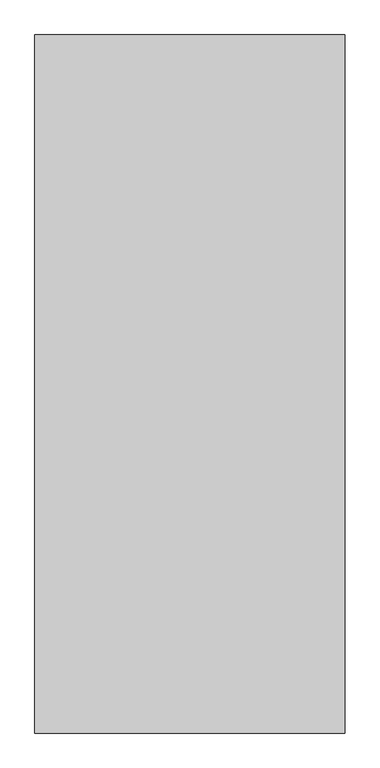
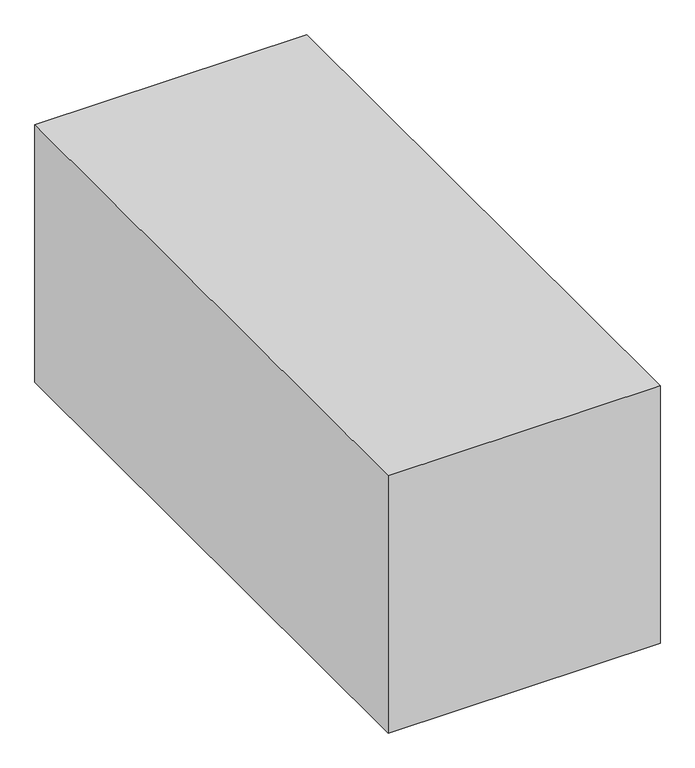
"""IFC4 building model written with IfcOpenShell, lengths in millimetres: proxy geometry, Space Planning Box_hec : Space Planning Box_hec."""

import ifcopenshell
import ifcopenshell.guid

model = None  # the IFC model being written
_history = None  # IfcOwnerHistory: only IFC2X3 demands one
_inside = {}  # id of a spatial element -> (the spatial element, [elements in it])
_under = {}  # id of a project, library or spatial element -> (it, [spatial elements below it])
_declared = {}  # id of a project -> (the project, [libraries it declares])
_typed = {}  # id of a type object -> (the type object, [elements of that type])
_made_of = {}  # id of a material, layer set ... -> (it, [elements and type objects made of it])


def new_model(schema):
    """Start an empty IFC model of exactly this schema.

    Asked for "IFC4X3", IfcOpenShell would pick the latest addendum, in which some entities
    have other attributes; the version numbers below select the first issue.
    IFC2X3 requires an IfcOwnerHistory on every rooted entity: one is made here for all.
    """
    global model, _history
    if schema == "IFC4X3":
        model = ifcopenshell.file(schema_version=(4, 3, 0, 0))
    else:
        model = ifcopenshell.file(schema=schema)
    _inside.clear()
    _under.clear()
    _declared.clear()
    _typed.clear()
    _made_of.clear()
    _history = None
    if model.schema == "IFC2X3":
        org = make("IfcOrganization", Name="unknown")
        user = make(
            "IfcPersonAndOrganization",
            ThePerson=make("IfcPerson", FamilyName="unknown"),
            TheOrganization=org,
        )
        app = make(
            "IfcApplication",
            ApplicationDeveloper=org,
            Version="unknown",
            ApplicationFullName="unknown",
            ApplicationIdentifier="unknown",
        )
        _history = make(
            "IfcOwnerHistory",
            OwningUser=user,
            OwningApplication=app,
            ChangeAction="ADDED",
            CreationDate=0,
        )
    return model


def make(cls, **values):
    """One entity of the class cls with the attributes given. An attribute that is None is left unset."""
    return model.create_entity(
        cls, **{name: value for name, value in values.items() if value is not None}
    )


def rooted(cls, **values):
    """An entity with a GlobalId (a new one), such as an element, a storey or a relation."""
    return make(cls, GlobalId=ifcopenshell.guid.new(), OwnerHistory=_history, **values)


def si_unit(unit_type, name, prefix=None):
    """IfcSIUnit, for example si_unit("LENGTHUNIT", "METRE", prefix="MILLI")."""
    return make("IfcSIUnit", UnitType=unit_type, Prefix=prefix, Name=name)


def assignment(units):
    """IfcUnitAssignment: the units of a project."""
    return None if units is None else make("IfcUnitAssignment", Units=units)


def point(xyz):
    """IfcCartesianPoint."""
    return None if xyz is None else make("IfcCartesianPoint", Coordinates=xyz)


def direction(xyz):
    """IfcDirection."""
    return None if xyz is None else make("IfcDirection", DirectionRatios=xyz)


def frame(location, z_axis=None, x_axis=None):
    """IfcAxis2Placement3D, a coordinate frame: its origin and axes. An axis left out is left unset."""
    return make(
        "IfcAxis2Placement3D",
        Location=point(location),
        Axis=direction(z_axis),
        RefDirection=direction(x_axis),
    )


def origin():
    """The frame at (0, 0, 0) with its axes left unset."""
    return frame((0.0, 0.0, 0.0))


def origin_with_axes():
    """The frame at (0, 0, 0) with the z axis (0, 0, 1) and the x axis (1, 0, 0) written out."""
    return frame((0.0, 0.0, 0.0), z_axis=(0.0, 0.0, 1.0), x_axis=(1.0, 0.0, 0.0))


def place(relative_to, where):
    """IfcLocalPlacement: puts the frame where relative to a parent placement (None: the world)."""
    return make(
        "IfcLocalPlacement", PlacementRelTo=relative_to, RelativePlacement=where
    )


def context(
    kind, dimensions, precision=None, world=None, true_north=None, identifier=None
):
    """IfcGeometricRepresentationContext, for example the 3D "Model" context."""
    return make(
        "IfcGeometricRepresentationContext",
        ContextIdentifier=identifier,
        ContextType=kind,
        CoordinateSpaceDimension=dimensions,
        Precision=precision,
        WorldCoordinateSystem=world,
        TrueNorth=true_north,
    )


def project(units=None, contexts=None):
    """IfcProject with its units and contexts."""
    return rooted(
        "IfcProject",
        Name="project",
        RepresentationContexts=contexts,
        UnitsInContext=assignment(units),
    )


def spatial(cls, under=None, at=None, **own):
    """A site, building, storey or space (cls), placed at a placement, below another one or the project."""
    s = rooted(cls, ObjectPlacement=at, **own)
    if under is not None:
        _under.setdefault(under.id(), (under, []))[1].append(s)
    return s


def polyline(points):
    """IfcPolyline through the points."""
    return make("IfcPolyline", Points=[point(p) for p in points])


def outline(outer, holes=None, kind="AREA"):
    """IfcArbitraryClosedProfileDef: a profile drawn as a closed curve; with holes, ...WithVoids."""
    if holes is None:
        return make("IfcArbitraryClosedProfileDef", ProfileType=kind, OuterCurve=outer)
    return make(
        "IfcArbitraryProfileDefWithVoids",
        ProfileType=kind,
        OuterCurve=outer,
        InnerCurves=holes,
    )


def extrude(swept, where, along, depth):
    """IfcExtrudedAreaSolid: the profile swept, set in the frame where, extruded along a direction by depth."""
    return make(
        "IfcExtrudedAreaSolid",
        SweptArea=swept,
        Position=where,
        ExtrudedDirection=direction(along),
        Depth=depth,
    )


def shape(context_of_items, identifier, shape_type, items):
    """IfcShapeRepresentation: the items that make up one representation, for example the "Body"."""
    return make(
        "IfcShapeRepresentation",
        ContextOfItems=context_of_items,
        RepresentationIdentifier=identifier,
        RepresentationType=shape_type,
        Items=items,
    )


def source(mapping_origin, context_of_items, identifier, shape_type, items):
    """IfcRepresentationMap: a shape defined once, which mapped items show again and again."""
    return make(
        "IfcRepresentationMap",
        MappingOrigin=mapping_origin,
        MappedRepresentation=shape(context_of_items, identifier, shape_type, items),
    )


def transform(
    local_origin,
    x_axis=None,
    y_axis=None,
    z_axis=None,
    scale=None,
    scale2=None,
    scale3=None,
    uniform=True,
):
    """IfcCartesianTransformationOperator3D, or its non-uniform kind. x_axis, y_axis, z_axis: its Axis1, 2, 3."""
    if uniform:
        return make(
            "IfcCartesianTransformationOperator3D",
            Axis1=direction(x_axis),
            Axis2=direction(y_axis),
            LocalOrigin=point(local_origin),
            Scale=scale,
            Axis3=direction(z_axis),
        )
    return make(
        "IfcCartesianTransformationOperator3DnonUniform",
        Axis1=direction(x_axis),
        Axis2=direction(y_axis),
        LocalOrigin=point(local_origin),
        Scale=scale,
        Axis3=direction(z_axis),
        Scale2=scale2,
        Scale3=scale3,
    )


def mapped(mapping_source, mapping_target):
    """IfcMappedItem: shows the shape of a source again, moved by a transform."""
    return make(
        "IfcMappedItem", MappingSource=mapping_source, MappingTarget=mapping_target
    )


def made_of(thing, what):
    """Note that an element or type object is made of a material, layer set ...; save() writes the relation."""
    if what is not None:
        _made_of.setdefault(what.id(), (what, []))[1].append(thing)
    return thing


def element(
    cls,
    number,
    at=None,
    inside=None,
    cuts=None,
    type_object=None,
    material=None,
    context=None,
    identifier="Body",
    shape_type=None,
    held_by="IfcProductDefinitionShape",
    body=None,
    shapes=None,
    **own,
):
    """One element of the class cls, such as IfcWall. Its Tag is "e" and its number.

    at: its placement. inside: the storey or other place that contains it. cuts: it is an
    opening in that element (IfcRelVoidsElement). A single representation is given by context,
    identifier, shape_type and body (its items); several are given by shapes. held_by: the class
    of the entity that holds the representations. save() writes the other relations.
    """
    e = rooted(cls, Tag="e%d" % number, ObjectPlacement=at, **own)
    if body is not None:
        shapes = [shape(context, identifier, shape_type, body)]
    if shapes is not None:
        e.Representation = make(held_by, Representations=shapes)
    if inside is not None:
        _inside.setdefault(inside.id(), (inside, []))[1].append(e)
    if cuts is not None:
        rooted(
            "IfcRelVoidsElement", RelatingBuildingElement=cuts, RelatedOpeningElement=e
        )
    if type_object is not None:
        _typed.setdefault(type_object.id(), (type_object, []))[1].append(e)
    return made_of(e, material)


def aggregate(whole, parts):
    """IfcRelAggregates: a whole, such as a stair, and the parts it consists of."""
    return rooted("IfcRelAggregates", RelatingObject=whole, RelatedObjects=parts)


def save(model, path):
    """Write the relations noted so far, then the file.

    IfcRelAggregates (storeys below a building ...), IfcRelContainedInSpatialStructure (elements
    in a storey), IfcRelDefinesByType, IfcRelAssociatesMaterial and IfcRelDeclares: one each for
    every whole, place, type object, material and project.
    """
    for whole, parts in _under.values():
        aggregate(whole, parts)
    for where, things in _inside.values():
        rooted(
            "IfcRelContainedInSpatialStructure",
            RelatedElements=things,
            RelatingStructure=where,
        )
    for kind, things in _typed.values():
        rooted("IfcRelDefinesByType", RelatedObjects=things, RelatingType=kind)
    for what, things in _made_of.values():
        rooted("IfcRelAssociatesMaterial", RelatedObjects=things, RelatingMaterial=what)
    for by, libraries in _declared.values():
        rooted("IfcRelDeclares", RelatingContext=by, RelatedDefinitions=libraries)
    model.write(path)


def generic_models_73802227(model_context):
    return source(origin(), model_context, "Body", "SweptSolid", [
        extrude(outline(polyline([(2000.0, 4500.0), (2000.0, -4500.0), (-2000.0, -4500.0), (-2000.0, 4500.0), (2000.0, 4500.0)])), origin_with_axes(), (0.0, 0.0, 1.0), 4000.0),
    ])


if __name__ == "__main__":
    model = new_model("IFC4")
    model_context = context("Model", 3, world=origin())
    ifc_project = project(units=[si_unit("LENGTHUNIT", "METRE", prefix="MILLI")], contexts=[model_context])
    site = spatial("IfcSite", under=ifc_project)
    building = spatial("IfcBuilding", under=site)
    placement = place(None, origin())
    generic_models_shape = generic_models_73802227(model_context)
    element("IfcBuildingElementProxy", 1, Name="Space Planning Box_hec : Space Planning Box_hec", ObjectType="Space Planning Box_hec : Space Planning Box_hec", at=placement, inside=building, context=model_context, shape_type="MappedRepresentation", body=[
        mapped(generic_models_shape, transform((0.0, 0.0, 0.0), x_axis=(1.0, 0.0, 0.0), y_axis=(0.0, 1.0, 0.0), z_axis=(0.0, 0.0, 1.0))),
    ])
    save(model, "model.ifc")

# Revit data of these elements
# Type "Space Planning Box_hec : Space Planning Box_hec"
#   Type Comments = "..."
#   Room Name [instance default] = "?"
#   Interior Finish [instance default] = ""
#   Exterior Finish [instance default] = ""
#   Department [instance default] = ""
#   Assembly Code = "..."
#   Width [instance default] = 1524 mm
#   Program Area [instance default] = 0 m²
#   Length [instance default] = 1524 mm
#   Height [instance default] = 1524 mm
#   Area [instance default] = 2.32258 m²
#   Fill Color [instance default] = Cyan
#   Default Elevation = 0
# Element 1 (IfcBuildingElementProxy, "Space Planning Box_hec : Space Planning Box_hec")
#   Room Name = "Stairway"
#   Interior Finish = "IF2"
#   Exterior Finish = "EF1"
#   Department = "EL"
#   Width = 4000 mm
#   Program Area = 36 m²
#   Length = 9000 mm
#   Height = 4000 mm
#   Area = 36 m²
#   Fill Color = Blue
#   Materials on its faces: "Blue"
# Materials
#   "Cyan": class "Generic", colour RGB 0 255 255, transparency 0.2, Cost = 0
#   "Blue": class "Generic", colour RGB 0 0 255, transparency 0.2, Cost = 0
